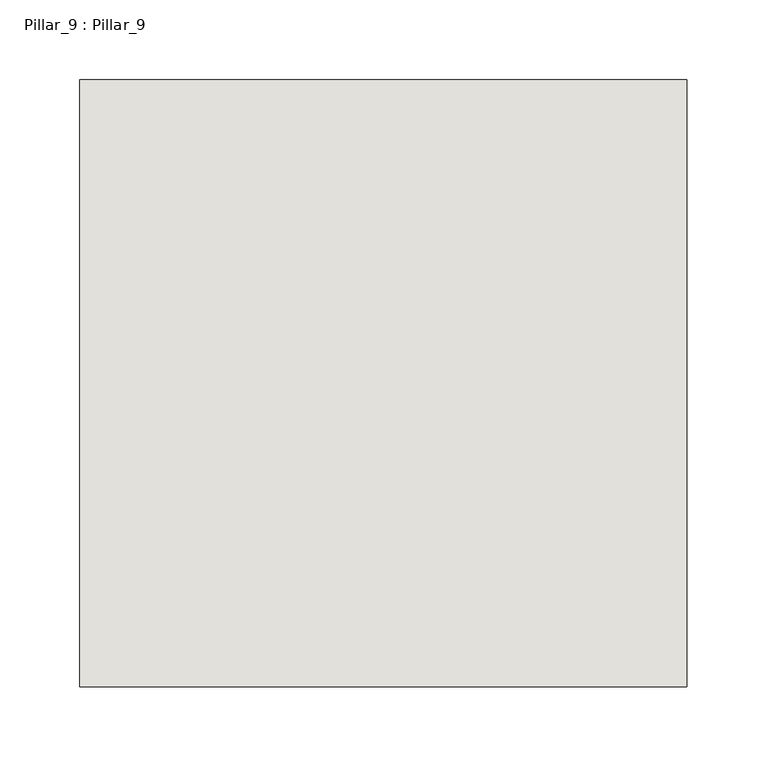
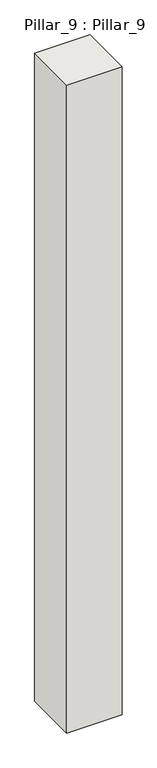
"""IFC4 building model written with IfcOpenShell, lengths in millimetres: wall geometry, Pillar_9 : Pillar_9."""

from ifc_helpers import new_model, si_unit, origin, origin_with_axes, place, context, project, spatial, polyline, outline, extrude, source, transform, mapped, element, save


def pillar_9_pillar_9_1ccd6465(model_context):
    return source(origin(), model_context, "Body", "SweptSolid", [
        extrude(outline(polyline([(5040.0, 3770.0), (4660.0, 3770.0), (4660.0, 4150.0), (5040.0, 4150.0), (5040.0, 3770.0)])), origin_with_axes(), (0.0, 0.0, 1.0), 4700.0),
    ])


if __name__ == "__main__":
    model = new_model("IFC4")
    model_context = context("Model", 3, world=origin())
    ifc_project = project(units=[si_unit("LENGTHUNIT", "METRE", prefix="MILLI")], contexts=[model_context])
    site = spatial("IfcSite", under=ifc_project)
    building = spatial("IfcBuilding", under=site)
    placement = place(None, origin())
    pillar_9_pillar_9_shape = pillar_9_pillar_9_1ccd6465(model_context)
    element("IfcWall", 1, ObjectType="Pillar_9 : Pillar_9", at=placement, inside=building, context=model_context, shape_type="MappedRepresentation", body=[
        mapped(pillar_9_pillar_9_shape, transform((0.0, 0.0, 0.0), x_axis=(1.0, 0.0, 0.0), y_axis=(0.0, 1.0, 0.0), z_axis=(0.0, 0.0, 1.0))),
    ])
    save(model, "model.ifc")

# Revit data of these elements
# Type "Pillar_9 : Pillar_9"
#   NameOverride = "Pillar_9"
# Element 1 (IfcWall, "Pillar_9 : Pillar_9")
#   Materials on its faces: "IfcSurfaceStyle #33"
# Materials
#   "IfcSurfaceStyle #33": class "Unassigned", colour RGB 214 214 214, transparency 0
